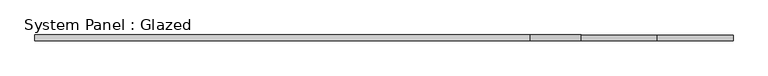
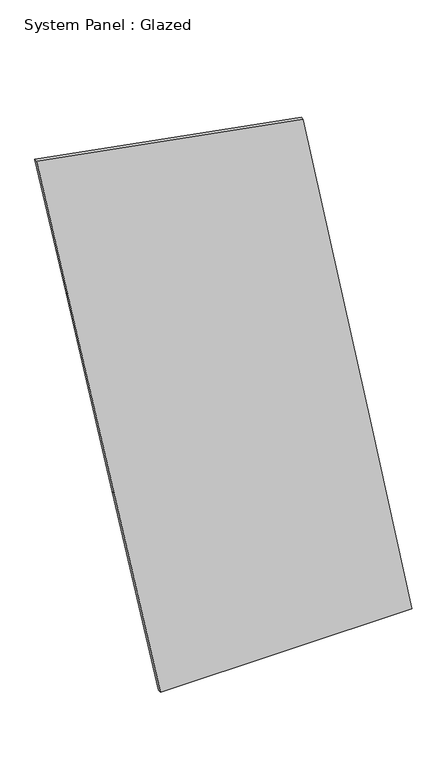
"""IFC4 building model written with IfcOpenShell, lengths in millimetres: plate geometry, System Panel : Glazed."""

from ifc_helpers import new_model, si_unit, frame, origin, place, context, project, spatial, polyline, outline, extrude, source, transform, mapped, element, save


def system_panel_glazed_86de8691(model_context):
    return source(origin(), model_context, "Body", "SweptSolid", [
        extrude(outline(polyline([(0.0, -508.5103179), (0.0, 1495.2866302), (1656.4702773, 1170.1496772), (3312.9405547, 845.0127241), (4423.4425676, 627.0400591), (4812.9687485, -1495.2866302), (3604.6764736, -1247.5571606), (1802.3382368, -878.0337392), (0.0, -508.5103179)])), frame((0.0, -49.5, 0.0), z_axis=(0.0, 1.0, 0.0), x_axis=(0.0, 0.0, 1.0)), (0.0, 0.0, 1.0), 25.0),
    ])


if __name__ == "__main__":
    model = new_model("IFC4")
    model_context = context("Model", 3, world=origin())
    ifc_project = project(units=[si_unit("LENGTHUNIT", "METRE", prefix="MILLI")], contexts=[model_context])
    site = spatial("IfcSite", under=ifc_project)
    building = spatial("IfcBuilding", under=site)
    placement = place(None, origin())
    system_panel_glazed_shape = system_panel_glazed_86de8691(model_context)
    element("IfcPlate", 1, ObjectType="System Panel : Glazed", at=placement, inside=building, context=model_context, shape_type="MappedRepresentation", body=[
        mapped(system_panel_glazed_shape, transform((0.0, 0.0, 0.0), x_axis=(1.0, 0.0, 0.0), y_axis=(0.0, 1.0, 0.0), z_axis=(0.0, 0.0, 1.0))),
    ])
    save(model, "model.ifc")

# Revit data of these elements
# Element 1 (IfcPlate, "System Panel : Glazed")
#   Materials on its faces: "Glass, Clear Glazing"
# Materials
#   "Glass, Clear Glazing": class "Glass", colour RGB 247 249 248, transparency 0.85, Description = "Clear glazing", Cost = 0
